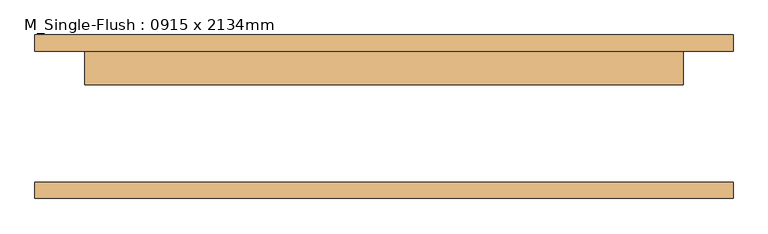
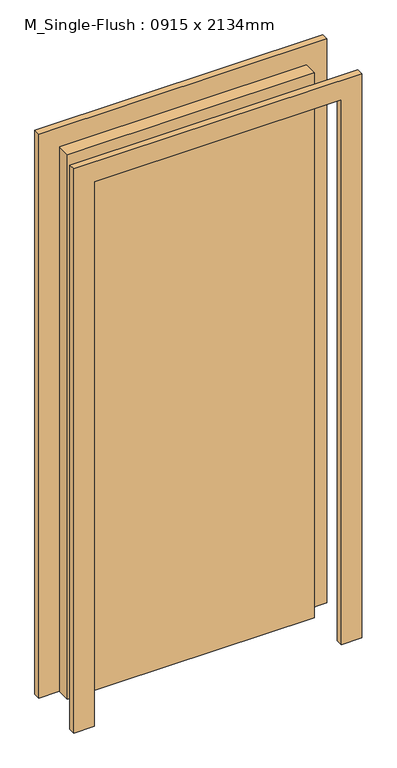
"""IFC4 building model written with IfcOpenShell, lengths in millimetres: door geometry, M_Single-Flush : 0915 x 2134mm."""

import ifcopenshell
import ifcopenshell.guid

model = None  # the IFC model being written
_history = None  # IfcOwnerHistory: only IFC2X3 demands one
_inside = {}  # id of a spatial element -> (the spatial element, [elements in it])
_under = {}  # id of a project, library or spatial element -> (it, [spatial elements below it])
_declared = {}  # id of a project -> (the project, [libraries it declares])
_typed = {}  # id of a type object -> (the type object, [elements of that type])
_made_of = {}  # id of a material, layer set ... -> (it, [elements and type objects made of it])


def new_model(schema):
    """Start an empty IFC model of exactly this schema.

    Asked for "IFC4X3", IfcOpenShell would pick the latest addendum, in which some entities
    have other attributes; the version numbers below select the first issue.
    IFC2X3 requires an IfcOwnerHistory on every rooted entity: one is made here for all.
    """
    global model, _history
    if schema == "IFC4X3":
        model = ifcopenshell.file(schema_version=(4, 3, 0, 0))
    else:
        model = ifcopenshell.file(schema=schema)
    _inside.clear()
    _under.clear()
    _declared.clear()
    _typed.clear()
    _made_of.clear()
    _history = None
    if model.schema == "IFC2X3":
        org = make("IfcOrganization", Name="unknown")
        user = make(
            "IfcPersonAndOrganization",
            ThePerson=make("IfcPerson", FamilyName="unknown"),
            TheOrganization=org,
        )
        app = make(
            "IfcApplication",
            ApplicationDeveloper=org,
            Version="unknown",
            ApplicationFullName="unknown",
            ApplicationIdentifier="unknown",
        )
        _history = make(
            "IfcOwnerHistory",
            OwningUser=user,
            OwningApplication=app,
            ChangeAction="ADDED",
            CreationDate=0,
        )
    return model


def make(cls, **values):
    """One entity of the class cls with the attributes given. An attribute that is None is left unset."""
    return model.create_entity(
        cls, **{name: value for name, value in values.items() if value is not None}
    )


def rooted(cls, **values):
    """An entity with a GlobalId (a new one), such as an element, a storey or a relation."""
    return make(cls, GlobalId=ifcopenshell.guid.new(), OwnerHistory=_history, **values)


def si_unit(unit_type, name, prefix=None):
    """IfcSIUnit, for example si_unit("LENGTHUNIT", "METRE", prefix="MILLI")."""
    return make("IfcSIUnit", UnitType=unit_type, Prefix=prefix, Name=name)


def assignment(units):
    """IfcUnitAssignment: the units of a project."""
    return None if units is None else make("IfcUnitAssignment", Units=units)


def point(xyz):
    """IfcCartesianPoint."""
    return None if xyz is None else make("IfcCartesianPoint", Coordinates=xyz)


def direction(xyz):
    """IfcDirection."""
    return None if xyz is None else make("IfcDirection", DirectionRatios=xyz)


def frame(location, z_axis=None, x_axis=None):
    """IfcAxis2Placement3D, a coordinate frame: its origin and axes. An axis left out is left unset."""
    return make(
        "IfcAxis2Placement3D",
        Location=point(location),
        Axis=direction(z_axis),
        RefDirection=direction(x_axis),
    )


def origin():
    """The frame at (0, 0, 0) with its axes left unset."""
    return frame((0.0, 0.0, 0.0))


def origin_with_axes():
    """The frame at (0, 0, 0) with the z axis (0, 0, 1) and the x axis (1, 0, 0) written out."""
    return frame((0.0, 0.0, 0.0), z_axis=(0.0, 0.0, 1.0), x_axis=(1.0, 0.0, 0.0))


def place(relative_to, where):
    """IfcLocalPlacement: puts the frame where relative to a parent placement (None: the world)."""
    return make(
        "IfcLocalPlacement", PlacementRelTo=relative_to, RelativePlacement=where
    )


def context(
    kind, dimensions, precision=None, world=None, true_north=None, identifier=None
):
    """IfcGeometricRepresentationContext, for example the 3D "Model" context."""
    return make(
        "IfcGeometricRepresentationContext",
        ContextIdentifier=identifier,
        ContextType=kind,
        CoordinateSpaceDimension=dimensions,
        Precision=precision,
        WorldCoordinateSystem=world,
        TrueNorth=true_north,
    )


def project(units=None, contexts=None):
    """IfcProject with its units and contexts."""
    return rooted(
        "IfcProject",
        Name="project",
        RepresentationContexts=contexts,
        UnitsInContext=assignment(units),
    )


def spatial(cls, under=None, at=None, **own):
    """A site, building, storey or space (cls), placed at a placement, below another one or the project."""
    s = rooted(cls, ObjectPlacement=at, **own)
    if under is not None:
        _under.setdefault(under.id(), (under, []))[1].append(s)
    return s


def polyline(points):
    """IfcPolyline through the points."""
    return make("IfcPolyline", Points=[point(p) for p in points])


def outline(outer, holes=None, kind="AREA"):
    """IfcArbitraryClosedProfileDef: a profile drawn as a closed curve; with holes, ...WithVoids."""
    if holes is None:
        return make("IfcArbitraryClosedProfileDef", ProfileType=kind, OuterCurve=outer)
    return make(
        "IfcArbitraryProfileDefWithVoids",
        ProfileType=kind,
        OuterCurve=outer,
        InnerCurves=holes,
    )


def extrude(swept, where, along, depth):
    """IfcExtrudedAreaSolid: the profile swept, set in the frame where, extruded along a direction by depth."""
    return make(
        "IfcExtrudedAreaSolid",
        SweptArea=swept,
        Position=where,
        ExtrudedDirection=direction(along),
        Depth=depth,
    )


def shape(context_of_items, identifier, shape_type, items):
    """IfcShapeRepresentation: the items that make up one representation, for example the "Body"."""
    return make(
        "IfcShapeRepresentation",
        ContextOfItems=context_of_items,
        RepresentationIdentifier=identifier,
        RepresentationType=shape_type,
        Items=items,
    )


def source(mapping_origin, context_of_items, identifier, shape_type, items):
    """IfcRepresentationMap: a shape defined once, which mapped items show again and again."""
    return make(
        "IfcRepresentationMap",
        MappingOrigin=mapping_origin,
        MappedRepresentation=shape(context_of_items, identifier, shape_type, items),
    )


def transform(
    local_origin,
    x_axis=None,
    y_axis=None,
    z_axis=None,
    scale=None,
    scale2=None,
    scale3=None,
    uniform=True,
):
    """IfcCartesianTransformationOperator3D, or its non-uniform kind. x_axis, y_axis, z_axis: its Axis1, 2, 3."""
    if uniform:
        return make(
            "IfcCartesianTransformationOperator3D",
            Axis1=direction(x_axis),
            Axis2=direction(y_axis),
            LocalOrigin=point(local_origin),
            Scale=scale,
            Axis3=direction(z_axis),
        )
    return make(
        "IfcCartesianTransformationOperator3DnonUniform",
        Axis1=direction(x_axis),
        Axis2=direction(y_axis),
        LocalOrigin=point(local_origin),
        Scale=scale,
        Axis3=direction(z_axis),
        Scale2=scale2,
        Scale3=scale3,
    )


def mapped(mapping_source, mapping_target):
    """IfcMappedItem: shows the shape of a source again, moved by a transform."""
    return make(
        "IfcMappedItem", MappingSource=mapping_source, MappingTarget=mapping_target
    )


def made_of(thing, what):
    """Note that an element or type object is made of a material, layer set ...; save() writes the relation."""
    if what is not None:
        _made_of.setdefault(what.id(), (what, []))[1].append(thing)
    return thing


def element(
    cls,
    number,
    at=None,
    inside=None,
    cuts=None,
    type_object=None,
    material=None,
    context=None,
    identifier="Body",
    shape_type=None,
    held_by="IfcProductDefinitionShape",
    body=None,
    shapes=None,
    **own,
):
    """One element of the class cls, such as IfcWall. Its Tag is "e" and its number.

    at: its placement. inside: the storey or other place that contains it. cuts: it is an
    opening in that element (IfcRelVoidsElement). A single representation is given by context,
    identifier, shape_type and body (its items); several are given by shapes. held_by: the class
    of the entity that holds the representations. save() writes the other relations.
    """
    e = rooted(cls, Tag="e%d" % number, ObjectPlacement=at, **own)
    if body is not None:
        shapes = [shape(context, identifier, shape_type, body)]
    if shapes is not None:
        e.Representation = make(held_by, Representations=shapes)
    if inside is not None:
        _inside.setdefault(inside.id(), (inside, []))[1].append(e)
    if cuts is not None:
        rooted(
            "IfcRelVoidsElement", RelatingBuildingElement=cuts, RelatedOpeningElement=e
        )
    if type_object is not None:
        _typed.setdefault(type_object.id(), (type_object, []))[1].append(e)
    return made_of(e, material)


def aggregate(whole, parts):
    """IfcRelAggregates: a whole, such as a stair, and the parts it consists of."""
    return rooted("IfcRelAggregates", RelatingObject=whole, RelatedObjects=parts)


def save(model, path):
    """Write the relations noted so far, then the file.

    IfcRelAggregates (storeys below a building ...), IfcRelContainedInSpatialStructure (elements
    in a storey), IfcRelDefinesByType, IfcRelAssociatesMaterial and IfcRelDeclares: one each for
    every whole, place, type object, material and project.
    """
    for whole, parts in _under.values():
        aggregate(whole, parts)
    for where, things in _inside.values():
        rooted(
            "IfcRelContainedInSpatialStructure",
            RelatedElements=things,
            RelatingStructure=where,
        )
    for kind, things in _typed.values():
        rooted("IfcRelDefinesByType", RelatedObjects=things, RelatingType=kind)
    for what, things in _made_of.values():
        rooted("IfcRelAssociatesMaterial", RelatedObjects=things, RelatingMaterial=what)
    for by, libraries in _declared.values():
        rooted("IfcRelDeclares", RelatingContext=by, RelatedDefinitions=libraries)
    model.write(path)


def m_single_flush_0915_x_2134mm_6a9e8738(model_context):
    return source(origin(), model_context, "Body", "SweptSolid", [
        extrude(outline(polyline([(2210.0, -533.5), (0.0, -533.5), (0.0, -457.5), (2134.0, -457.5), (2134.0, 457.5), (0.0, 457.5), (0.0, 533.5), (2210.0, 533.5), (2210.0, -533.5)])), frame((0.0, 100.0, 0.0), z_axis=(0.0, 1.0, 0.0), x_axis=(0.0, 0.0, 1.0)), (0.0, 0.0, 1.0), 25.0),
        extrude(outline(polyline([(2210.0, 533.5), (2210.0, -533.5), (0.0, -533.5), (0.0, -457.5), (2134.0, -457.5), (2134.0, 457.5), (0.0, 457.5), (0.0, 533.5), (2210.0, 533.5)])), frame((0.0, -125.0, 0.0), z_axis=(0.0, 1.0, 0.0), x_axis=(0.0, 0.0, 1.0)), (0.0, 0.0, 1.0), 25.0),
        extrude(outline(polyline([(457.5, 49.0), (-457.5, 49.0), (-457.5, 100.0), (457.5, 100.0), (457.5, 49.0)])), origin_with_axes(), (0.0, 0.0, 1.0), 2134.0),
    ])


if __name__ == "__main__":
    model = new_model("IFC4")
    model_context = context("Model", 3, world=origin())
    ifc_project = project(units=[si_unit("LENGTHUNIT", "METRE", prefix="MILLI")], contexts=[model_context])
    site = spatial("IfcSite", under=ifc_project)
    building = spatial("IfcBuilding", under=site)
    placement = place(None, origin())
    m_single_flush_0915_x_2134mm_shape = m_single_flush_0915_x_2134mm_6a9e8738(model_context)
    element("IfcDoor", 1, ObjectType="M_Single-Flush : 0915 x 2134mm", at=placement, inside=building, context=model_context, shape_type="MappedRepresentation", body=[
        mapped(m_single_flush_0915_x_2134mm_shape, transform((0.0, 0.0, 0.0), x_axis=(1.0, 0.0, 0.0), y_axis=(0.0, 1.0, 0.0), z_axis=(0.0, 0.0, 1.0))),
    ])
    save(model, "model.ifc")

# Revit data of these elements
# Type "M_Single-Flush : 0915 x 2134mm"
#   Type Mark = "15"
#   Construction Type Id = "MDOOR"
#   Analytic Construction = "Metal"
#   Thickness = 0' - 2.00787"
#   Thermal Resistance (R) = 0.270117 (m²·K)/W
#   Heat Transfer Coefficient (U) = 3.7021 W/(m²·K)
#   Height = 7' - 0.01575"
#   Trim Projection Ext = 0' - 0.98425"
#   Trim Projection Int = 0' - 0.98425"
#   Trim Width = 0' - 2.99213"
#   Width = 3' - 0.02362"
#   Door Material = Door - Panel
#   Frame Material = Door - Frame
#   Visual Light Transmittance = 0
#   Solar Heat Gain Coefficient = 0
#   Function = (empty or 0)
#   Wall Closure = (empty or 0)
# Element 1 (IfcDoor, "M_Single-Flush : 0915 x 2134mm")
#   Materials on its faces: "Door - Frame", "Door - Panel"
# Materials
#   "Door - Panel": class "Wood", colour RGB 210 159 95, transparency 0, Cost = 0
#   "Door - Frame": class "Miscellaneous", colour RGB 118 70 51, transparency 0, Cost = 0
